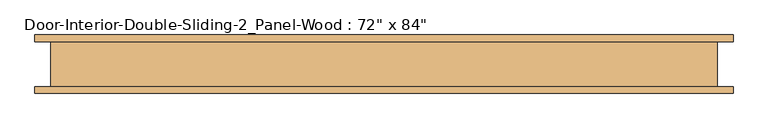
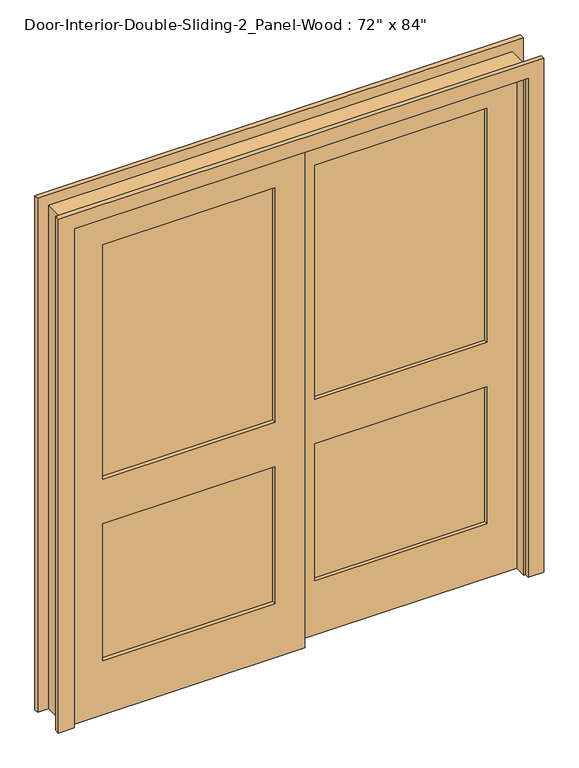
"""IFC4 building model written with IfcOpenShell, lengths in millimetres: door geometry."""

import ifcopenshell
import ifcopenshell.guid

model = None  # the IFC model being written
_history = None  # IfcOwnerHistory: only IFC2X3 demands one
_inside = {}  # id of a spatial element -> (the spatial element, [elements in it])
_under = {}  # id of a project, library or spatial element -> (it, [spatial elements below it])
_declared = {}  # id of a project -> (the project, [libraries it declares])
_typed = {}  # id of a type object -> (the type object, [elements of that type])
_made_of = {}  # id of a material, layer set ... -> (it, [elements and type objects made of it])


def new_model(schema):
    """Start an empty IFC model of exactly this schema.

    Asked for "IFC4X3", IfcOpenShell would pick the latest addendum, in which some entities
    have other attributes; the version numbers below select the first issue.
    IFC2X3 requires an IfcOwnerHistory on every rooted entity: one is made here for all.
    """
    global model, _history
    if schema == "IFC4X3":
        model = ifcopenshell.file(schema_version=(4, 3, 0, 0))
    else:
        model = ifcopenshell.file(schema=schema)
    _inside.clear()
    _under.clear()
    _declared.clear()
    _typed.clear()
    _made_of.clear()
    _history = None
    if model.schema == "IFC2X3":
        org = make("IfcOrganization", Name="unknown")
        user = make(
            "IfcPersonAndOrganization",
            ThePerson=make("IfcPerson", FamilyName="unknown"),
            TheOrganization=org,
        )
        app = make(
            "IfcApplication",
            ApplicationDeveloper=org,
            Version="unknown",
            ApplicationFullName="unknown",
            ApplicationIdentifier="unknown",
        )
        _history = make(
            "IfcOwnerHistory",
            OwningUser=user,
            OwningApplication=app,
            ChangeAction="ADDED",
            CreationDate=0,
        )
    return model


def make(cls, **values):
    """One entity of the class cls with the attributes given. An attribute that is None is left unset."""
    return model.create_entity(
        cls, **{name: value for name, value in values.items() if value is not None}
    )


def rooted(cls, **values):
    """An entity with a GlobalId (a new one), such as an element, a storey or a relation."""
    return make(cls, GlobalId=ifcopenshell.guid.new(), OwnerHistory=_history, **values)


def si_unit(unit_type, name, prefix=None):
    """IfcSIUnit, for example si_unit("LENGTHUNIT", "METRE", prefix="MILLI")."""
    return make("IfcSIUnit", UnitType=unit_type, Prefix=prefix, Name=name)


def assignment(units):
    """IfcUnitAssignment: the units of a project."""
    return None if units is None else make("IfcUnitAssignment", Units=units)


def point(xyz):
    """IfcCartesianPoint."""
    return None if xyz is None else make("IfcCartesianPoint", Coordinates=xyz)


def direction(xyz):
    """IfcDirection."""
    return None if xyz is None else make("IfcDirection", DirectionRatios=xyz)


def frame(location, z_axis=None, x_axis=None):
    """IfcAxis2Placement3D, a coordinate frame: its origin and axes. An axis left out is left unset."""
    return make(
        "IfcAxis2Placement3D",
        Location=point(location),
        Axis=direction(z_axis),
        RefDirection=direction(x_axis),
    )


def origin():
    """The frame at (0, 0, 0) with its axes left unset."""
    return frame((0.0, 0.0, 0.0))


def place(relative_to, where):
    """IfcLocalPlacement: puts the frame where relative to a parent placement (None: the world)."""
    return make(
        "IfcLocalPlacement", PlacementRelTo=relative_to, RelativePlacement=where
    )


def context(
    kind, dimensions, precision=None, world=None, true_north=None, identifier=None
):
    """IfcGeometricRepresentationContext, for example the 3D "Model" context."""
    return make(
        "IfcGeometricRepresentationContext",
        ContextIdentifier=identifier,
        ContextType=kind,
        CoordinateSpaceDimension=dimensions,
        Precision=precision,
        WorldCoordinateSystem=world,
        TrueNorth=true_north,
    )


def project(units=None, contexts=None):
    """IfcProject with its units and contexts."""
    return rooted(
        "IfcProject",
        Name="project",
        RepresentationContexts=contexts,
        UnitsInContext=assignment(units),
    )


def spatial(cls, under=None, at=None, **own):
    """A site, building, storey or space (cls), placed at a placement, below another one or the project."""
    s = rooted(cls, ObjectPlacement=at, **own)
    if under is not None:
        _under.setdefault(under.id(), (under, []))[1].append(s)
    return s


def polyline(points):
    """IfcPolyline through the points."""
    return make("IfcPolyline", Points=[point(p) for p in points])


def outline(outer, holes=None, kind="AREA"):
    """IfcArbitraryClosedProfileDef: a profile drawn as a closed curve; with holes, ...WithVoids."""
    if holes is None:
        return make("IfcArbitraryClosedProfileDef", ProfileType=kind, OuterCurve=outer)
    return make(
        "IfcArbitraryProfileDefWithVoids",
        ProfileType=kind,
        OuterCurve=outer,
        InnerCurves=holes,
    )


def extrude(swept, where, along, depth):
    """IfcExtrudedAreaSolid: the profile swept, set in the frame where, extruded along a direction by depth."""
    return make(
        "IfcExtrudedAreaSolid",
        SweptArea=swept,
        Position=where,
        ExtrudedDirection=direction(along),
        Depth=depth,
    )


def shape(context_of_items, identifier, shape_type, items):
    """IfcShapeRepresentation: the items that make up one representation, for example the "Body"."""
    return make(
        "IfcShapeRepresentation",
        ContextOfItems=context_of_items,
        RepresentationIdentifier=identifier,
        RepresentationType=shape_type,
        Items=items,
    )


def source(mapping_origin, context_of_items, identifier, shape_type, items):
    """IfcRepresentationMap: a shape defined once, which mapped items show again and again."""
    return make(
        "IfcRepresentationMap",
        MappingOrigin=mapping_origin,
        MappedRepresentation=shape(context_of_items, identifier, shape_type, items),
    )


def transform(
    local_origin,
    x_axis=None,
    y_axis=None,
    z_axis=None,
    scale=None,
    scale2=None,
    scale3=None,
    uniform=True,
):
    """IfcCartesianTransformationOperator3D, or its non-uniform kind. x_axis, y_axis, z_axis: its Axis1, 2, 3."""
    if uniform:
        return make(
            "IfcCartesianTransformationOperator3D",
            Axis1=direction(x_axis),
            Axis2=direction(y_axis),
            LocalOrigin=point(local_origin),
            Scale=scale,
            Axis3=direction(z_axis),
        )
    return make(
        "IfcCartesianTransformationOperator3DnonUniform",
        Axis1=direction(x_axis),
        Axis2=direction(y_axis),
        LocalOrigin=point(local_origin),
        Scale=scale,
        Axis3=direction(z_axis),
        Scale2=scale2,
        Scale3=scale3,
    )


def mapped(mapping_source, mapping_target):
    """IfcMappedItem: shows the shape of a source again, moved by a transform."""
    return make(
        "IfcMappedItem", MappingSource=mapping_source, MappingTarget=mapping_target
    )


def made_of(thing, what):
    """Note that an element or type object is made of a material, layer set ...; save() writes the relation."""
    if what is not None:
        _made_of.setdefault(what.id(), (what, []))[1].append(thing)
    return thing


def element(
    cls,
    number,
    at=None,
    inside=None,
    cuts=None,
    type_object=None,
    material=None,
    context=None,
    identifier="Body",
    shape_type=None,
    held_by="IfcProductDefinitionShape",
    body=None,
    shapes=None,
    **own,
):
    """One element of the class cls, such as IfcWall. Its Tag is "e" and its number.

    at: its placement. inside: the storey or other place that contains it. cuts: it is an
    opening in that element (IfcRelVoidsElement). A single representation is given by context,
    identifier, shape_type and body (its items); several are given by shapes. held_by: the class
    of the entity that holds the representations. save() writes the other relations.
    """
    e = rooted(cls, Tag="e%d" % number, ObjectPlacement=at, **own)
    if body is not None:
        shapes = [shape(context, identifier, shape_type, body)]
    if shapes is not None:
        e.Representation = make(held_by, Representations=shapes)
    if inside is not None:
        _inside.setdefault(inside.id(), (inside, []))[1].append(e)
    if cuts is not None:
        rooted(
            "IfcRelVoidsElement", RelatingBuildingElement=cuts, RelatedOpeningElement=e
        )
    if type_object is not None:
        _typed.setdefault(type_object.id(), (type_object, []))[1].append(e)
    return made_of(e, material)


def aggregate(whole, parts):
    """IfcRelAggregates: a whole, such as a stair, and the parts it consists of."""
    return rooted("IfcRelAggregates", RelatingObject=whole, RelatedObjects=parts)


def save(model, path):
    """Write the relations noted so far, then the file.

    IfcRelAggregates (storeys below a building ...), IfcRelContainedInSpatialStructure (elements
    in a storey), IfcRelDefinesByType, IfcRelAssociatesMaterial and IfcRelDeclares: one each for
    every whole, place, type object, material and project.
    """
    for whole, parts in _under.values():
        aggregate(whole, parts)
    for where, things in _inside.values():
        rooted(
            "IfcRelContainedInSpatialStructure",
            RelatedElements=things,
            RelatingStructure=where,
        )
    for kind, things in _typed.values():
        rooted("IfcRelDefinesByType", RelatedObjects=things, RelatingType=kind)
    for what, things in _made_of.values():
        rooted("IfcRelAssociatesMaterial", RelatedObjects=things, RelatingMaterial=what)
    for by, libraries in _declared.values():
        rooted("IfcRelDeclares", RelatingContext=by, RelatedDefinitions=libraries)
    model.write(path)


def door_670f2e89(model_context):
    return source(origin(), model_context, "Body", "SweptSolid", [
        extrude(outline(polyline([(793.75, 24.3416667), (793.75, 7.4083333), (95.25, 7.4083333), (95.25, 24.3416667), (793.75, 24.3416667)])), frame((0.0, 0.0, 1009.65), z_axis=(0.0, 0.0, 1.0), x_axis=(1.0, 0.0, 0.0)), (0.0, 0.0, 1.0), 1004.8875),
        extrude(outline(polyline([(793.75, 24.3416667), (793.75, 7.4083333), (95.25, 7.4083333), (95.25, 24.3416667), (793.75, 24.3416667)])), frame((0.0, 0.0, 231.775), z_axis=(0.0, 0.0, 1.0), x_axis=(1.0, 0.0, 0.0)), (0.0, 0.0, 1.0), 587.375),
        extrude(outline(polyline([(2133.6, -25.4), (0.0, -25.4), (0.0, 914.4), (2133.6, 914.4), (2133.6, -25.4)]), holes=[polyline([(2014.5375, 95.25), (2014.5375, 793.75), (1009.65, 793.75), (1009.65, 95.25), (2014.5375, 95.25)]), polyline([(819.15, 95.25), (819.15, 793.75), (231.775, 793.75), (231.775, 95.25), (819.15, 95.25)])]), frame((0.0, -9.525, 0.0), z_axis=(0.0, 1.0, 0.0), x_axis=(0.0, 0.0, 1.0)), (0.0, 0.0, 1.0), 50.8),
        extrude(outline(polyline([(-95.25, -26.4583333), (-95.25, -43.3916667), (-793.75, -43.3916667), (-793.75, -26.4583333), (-95.25, -26.4583333)])), frame((0.0, 0.0, 1009.65), z_axis=(0.0, 0.0, 1.0), x_axis=(1.0, 0.0, 0.0)), (0.0, 0.0, 1.0), 1004.8875),
        extrude(outline(polyline([(-95.25, -26.4583333), (-95.25, -43.3916667), (-793.75, -43.3916667), (-793.75, -26.4583333), (-95.25, -26.4583333)])), frame((0.0, 0.0, 231.775), z_axis=(0.0, 0.0, 1.0), x_axis=(1.0, 0.0, 0.0)), (0.0, 0.0, 1.0), 587.375),
        extrude(outline(polyline([(2133.6, -914.4), (0.0, -914.4), (0.0, 25.4), (2133.6, 25.4), (2133.6, -914.4)]), holes=[polyline([(2014.5375, -793.75), (2014.5375, -95.25), (1009.65, -95.25), (1009.65, -793.75), (2014.5375, -793.75)]), polyline([(819.15, -793.75), (819.15, -95.25), (231.775, -95.25), (231.775, -793.75), (819.15, -793.75)])]), frame((0.0, -60.325, 0.0), z_axis=(0.0, 1.0, 0.0), x_axis=(0.0, 0.0, 1.0)), (0.0, 0.0, 1.0), 50.8),
        extrude(outline(polyline([(0.0, 939.8), (2159.0, 939.8), (2159.0, -939.8), (0.0, -939.8), (0.0, -914.4), (2133.6, -914.4), (2133.6, 914.4), (0.0, 914.4), (0.0, 939.8)])), frame((0.0, -60.325, 0.0), z_axis=(0.0, 1.0, 0.0), x_axis=(0.0, 0.0, 1.0)), (0.0, 0.0, 1.0), 127.0),
        extrude(outline(polyline([(0.0, 984.25), (2203.45, 984.25), (2203.45, -984.25), (0.0, -984.25), (0.0, -920.75), (2139.95, -920.75), (2139.95, 920.75), (0.0, 920.75), (0.0, 984.25)])), frame((0.0, 66.675, 0.0), z_axis=(0.0, 1.0, 0.0), x_axis=(0.0, 0.0, 1.0)), (0.0, 0.0, 1.0), 19.05),
        extrude(outline(polyline([(0.0, 984.25), (2203.45, 984.25), (2203.45, -984.25), (0.0, -984.25), (0.0, -920.75), (2139.95, -920.75), (2139.95, 920.75), (0.0, 920.75), (0.0, 984.25)])), frame((0.0, -79.375, 0.0), z_axis=(0.0, 1.0, 0.0), x_axis=(0.0, 0.0, 1.0)), (0.0, 0.0, 1.0), 19.05),
    ])


if __name__ == "__main__":
    model = new_model("IFC4")
    model_context = context("Model", 3, world=origin())
    ifc_project = project(units=[si_unit("LENGTHUNIT", "METRE", prefix="MILLI")], contexts=[model_context])
    site = spatial("IfcSite", under=ifc_project)
    building = spatial("IfcBuilding", under=site)
    placement = place(None, origin())
    door_shape = door_670f2e89(model_context)
    element("IfcDoor", 1, ObjectType="Door-Interior-Double-Sliding-2_Panel-Wood : 72\" x 84\"", at=placement, inside=building, context=model_context, shape_type="MappedRepresentation", body=[
        mapped(door_shape, transform((0.0, 0.0, 0.0), x_axis=(1.0, 0.0, 0.0), y_axis=(0.0, 1.0, 0.0), z_axis=(0.0, 0.0, 1.0))),
    ])
    save(model, "model.ifc")

# Revit data of these elements
# Type "Door-Interior-Double-Sliding-2_Panel-Wood : 72\" x 84\""
#   Type Mark = "8"
#   Assembly Code = "C1020"
#   Analytic Construction = "Wooden"
#   Top Rail = 0' - 4 11/16"
#   Thickness = 0' - 2"
#   Thermal Resistance (R) = 2.5876 (h·ft²·°F)/BTU
#   Stiles = 0' - 4 3/4"
#   Rough Width = 6' - 2"
#   Rough Height = 7' - 1"
#   Lock Rail = 0' - 7 1/2"
#   Heat Transfer Coefficient (U) = 0.3865 BTU/(h·ft²·°F)
#   Bottom Rail = 0' - 9 1/8"
#   Height = 7' - 0"
#   Width = 6' - 0"
#   Define Thermal Properties by = 1
#   Trim Material = Cherry
#   Panel Material = Cherry
#   Frame Material = Door - Frame
#   Visual Light Transmittance = 0
#   Solar Heat Gain Coefficient = 0
#   Function = (empty or 0)
#   Wall Closure = (empty or 0)
# Element 1 (IfcDoor, "Door-Interior-Double-Sliding-2_Panel-Wood : 72\" x 84\"")
#   Materials on its faces: "Cherry", "Door - Frame"
# Materials
#   "Cherry": class "Wood", colour RGB 157 77 38, transparency 0, Description = "Prunus Serotina", Cost = 0
#   "Door - Frame": class "Unassigned", colour RGB 118 70 51, transparency 0
